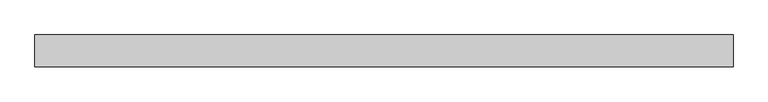
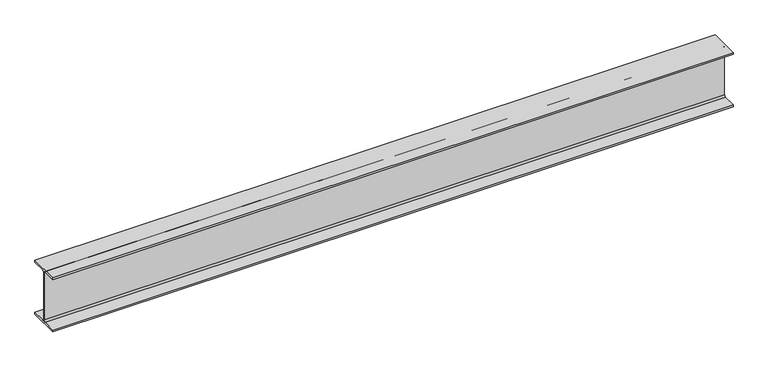
"""IFC4 building model written with IfcOpenShell, lengths in millimetres: beam geometry, Old_Steel Beam_H-KSD3502 : H_SB_ASB_H-340×250x9x14."""

from ifc_helpers import new_model, si_unit, point, frame, frame_2d, origin, place, context, project, spatial, polyline, circle_curve, trimmed, segment, composite_curve, outline, extrude, source, transform, mapped, element, save


def beam_b6deedb5(model_context):
    return source(origin(), model_context, "Body", "SweptSolid", [
        extrude(outline(composite_curve([segment(polyline([(82.5, -141.5), (82.5, -151.7), (-82.5, -151.7), (-82.5, -141.5), (-11.9, -141.5)]), True, "CONTINUOUS"), segment(trimmed(circle_curve(frame_2d((-11.9, -132.6)), 8.9), [point((-11.9, -141.5))], [point((-3.0, -132.6))], True, "CARTESIAN"), True, "CONTINUOUS"), segment(polyline([(-3.0, -132.6), (-3.0, 132.6)]), True, "CONTINUOUS"), segment(trimmed(circle_curve(frame_2d((-11.9, 132.6)), 8.9), [point((-3.0, 132.6))], [point((-11.9, 141.5))], True, "CARTESIAN"), True, "CONTINUOUS"), segment(polyline([(-11.9, 141.5), (-82.5, 141.5), (-82.5, 151.7), (82.5, 151.7), (82.5, 141.5), (11.9, 141.5)]), True, "CONTINUOUS"), segment(trimmed(circle_curve(frame_2d((11.9, 132.6)), 8.9), [point((11.9, 141.5))], [point((3.0, 132.6))], True, "CARTESIAN"), True, "CONTINUOUS"), segment(polyline([(3.0, 132.6), (3.0, -132.6)]), True, "CONTINUOUS"), segment(trimmed(circle_curve(frame_2d((11.9, -132.6)), 8.9), [point((3.0, -132.6))], [point((11.9, -141.5))], True, "CARTESIAN"), True, "CONTINUOUS"), segment(polyline([(11.9, -141.5), (82.5, -141.5)]), True, "CONTINUOUS")], self_intersect=False)), frame((-1812.3, 0.0, 0.0), z_axis=(1.0, 0.0, 0.0), x_axis=(0.0, 1.0, 0.0)), (0.0, 0.0, 1.0), 3624.6),
    ])


if __name__ == "__main__":
    model = new_model("IFC4")
    model_context = context("Model", 3, world=origin())
    ifc_project = project(units=[si_unit("LENGTHUNIT", "METRE", prefix="MILLI")], contexts=[model_context])
    site = spatial("IfcSite", under=ifc_project)
    building = spatial("IfcBuilding", under=site)
    placement = place(None, origin())
    beam_shape = beam_b6deedb5(model_context)
    element("IfcBeam", 1, ObjectType="Old_Steel Beam_H-KSD3502 : H_SB_ASB_H-340×250x9x14", at=placement, inside=building, context=model_context, shape_type="MappedRepresentation", body=[
        mapped(beam_shape, transform((0.0, 0.0, 0.0), x_axis=(1.0, 0.0, 0.0), y_axis=(0.0, 1.0, 0.0), z_axis=(0.0, 0.0, 1.0))),
    ])
    save(model, "model.ifc")

# Revit data of these elements
# Type "Old_Steel Beam_H-KSD3502 : H_SB_ASB_H-340×250x9x14"
#   Width = 25.0 cm
#   Web Thickness = 0.9 cm
#   Web Fillet = 2.0 cm
#   Warping Constant = 968661.0 cm⁶
#   Torsional Moment of Inertia = 53.6551 cm⁴
#   Torsional Modulus = 1.0 cm³
#   Section Area = 101.5 cm²
#   Plastic Modulus weak axis = 447.0 cm³
#   Plastic Modulus strong axis = 1410.0 cm³
#   Perimeter = 1.63 m²/m
#   Nominal Weight = 79.70 kgf/m
#   Moment of Inertia weak axis = 3650.00 cm⁴
#   Moment of Inertia strong axis = 21700.00 cm⁴
#   Height = 34.0 cm
#   Flange Thickness = 1.4 cm
#   Elastic Modulus weak axis = 292.0 cm³
#   Elastic Modulus strong axis = 1280.0 cm³
#   Centroid Vertical = 17.0 cm
#   Centroid Horizontal = 12.5 cm
#   Length [instance default] = 1.5240 m
#   Structural Material [instance default] = Steel, 45-345
#   Assembly Code = ""
# Element 1 (IfcBeam, "Old_Steel Beam_H-KSD3502 : H_SB_ASB_H-340×250x9x14")
#   Structural Material = none
# Materials
#   "Steel, 45-345": class "Metal", colour RGB 189 187 185, transparency 0, Description = "Steel 345 MPa", Cost = 0
